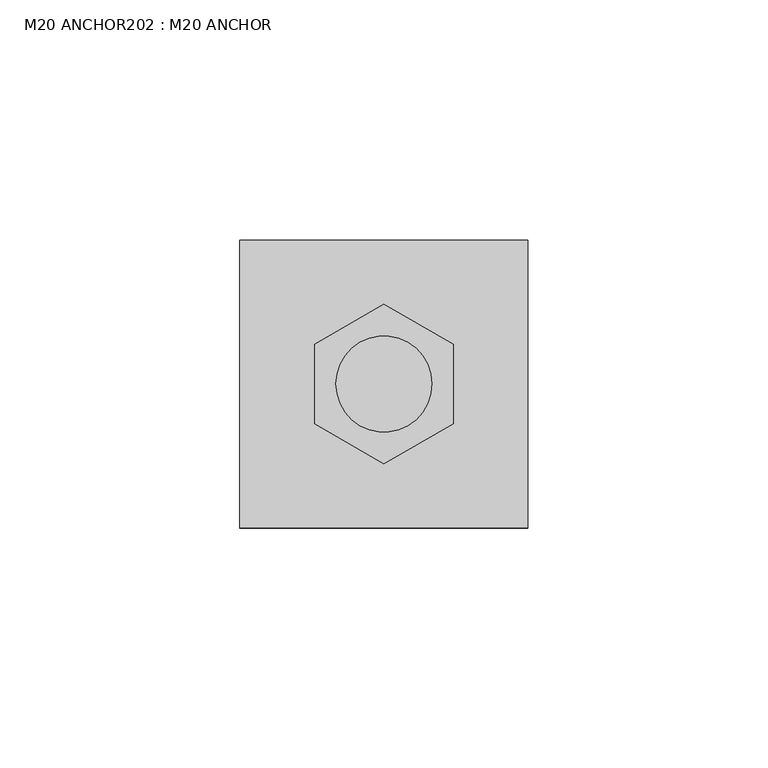
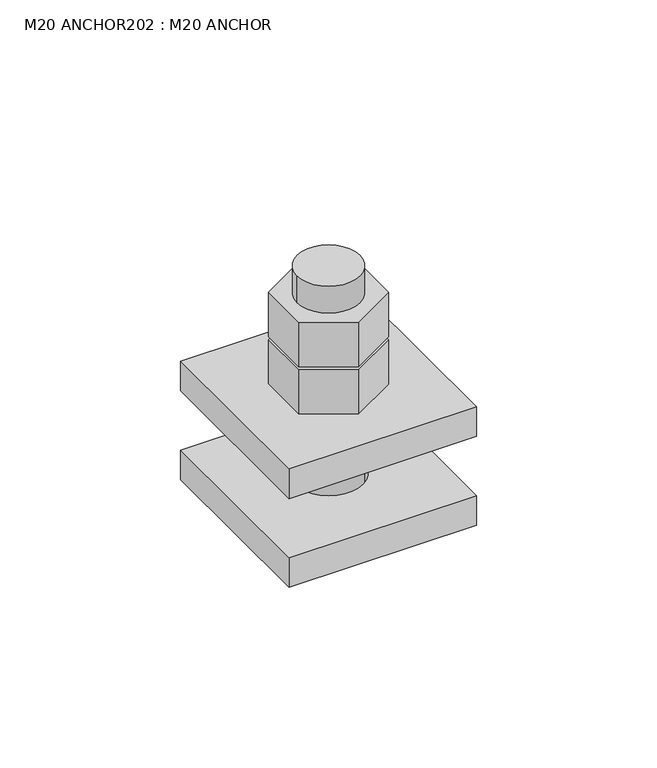
"""IFC4 building model written with IfcOpenShell, lengths in millimetres: fastener geometry, M20 ANCHOR202 : M20 ANCHOR."""

from ifc_helpers import new_model, si_unit, point, frame, frame_2d, origin, place, context, project, spatial, polyline, circle_curve, trimmed, segment, composite_curve, outline, extrude, source, transform, mapped, element, save


def m20_anchor202_m20_anchor_9b2e2336(model_context):
    return source(origin(), model_context, "Body", "SweptSolid", [
        extrude(outline(polyline([(8991.9144032, 22453.9464399), (8977.5062842, 22445.6279085), (8963.0981652, 22453.9464399), (8963.0981652, 22470.5835027), (8977.5062842, 22478.9020341), (8991.9144032, 22470.5835027), (8991.9144032, 22453.9464399)]), holes=[composite_curve([segment(trimmed(circle_curve(frame_2d((8977.5062842, 22462.2649713)), 10.0), [point((8967.5062842, 22462.2649713))], [point((8987.5062842, 22462.2649713))], True, "CARTESIAN"), True, "CONTINUOUS"), segment(trimmed(circle_curve(frame_2d((8977.5062842, 22462.2649713)), 10.0), [point((8987.5062842, 22462.2649713))], [point((8967.5062842, 22462.2649713))], True, "CARTESIAN"), True, "CONTINUOUS")], self_intersect=False)]), frame((0.0, 0.0, 246.0), z_axis=(0.0, 0.0, 1.0), x_axis=(1.0, 0.0, 0.0)), (0.0, 0.0, 1.0), 15.0),
        extrude(outline(polyline([(8991.9144032, 22453.9464399), (8977.5062842, 22445.6279085), (8963.0981652, 22453.9464399), (8963.0981652, 22470.5835027), (8977.5062842, 22478.9020341), (8991.9144032, 22470.5835027), (8991.9144032, 22453.9464399)]), holes=[composite_curve([segment(trimmed(circle_curve(frame_2d((8977.5062842, 22462.2649713)), 10.0), [point((8967.5062842, 22462.2649713))], [point((8987.5062842, 22462.2649713))], True, "CARTESIAN"), True, "CONTINUOUS"), segment(trimmed(circle_curve(frame_2d((8977.5062842, 22462.2649713)), 10.0), [point((8987.5062842, 22462.2649713))], [point((8967.5062842, 22462.2649713))], True, "CARTESIAN"), True, "CONTINUOUS")], self_intersect=False)]), frame((0.0, 0.0, 230.0), z_axis=(0.0, 0.0, 1.0), x_axis=(1.0, 0.0, 0.0)), (0.0, 0.0, 1.0), 15.0),
        extrude(outline(composite_curve([segment(trimmed(circle_curve(frame_2d((8977.5062842, 22462.2649713)), 10.0), [point((8967.5062842, 22462.2649713))], [point((8987.5062842, 22462.2649713))], False, "CARTESIAN"), True, "CONTINUOUS"), segment(trimmed(circle_curve(frame_2d((8977.5062842, 22462.2649713)), 10.0), [point((8987.5062842, 22462.2649713))], [point((8967.5062842, 22462.2649713))], False, "CARTESIAN"), True, "CONTINUOUS")], self_intersect=False)), frame((0.0, 0.0, 190.0), z_axis=(0.0, 0.0, 1.0), x_axis=(1.0, 0.0, 0.0)), (0.0, 0.0, 1.0), 80.0),
        extrude(outline(polyline([(9007.5062842, 22432.2649713), (8947.5062842, 22432.2649713), (8947.5062842, 22492.2649713), (9007.5062842, 22492.2649713), (9007.5062842, 22432.2649713)]), holes=[composite_curve([segment(trimmed(circle_curve(frame_2d((8977.5062842, 22462.2649713)), 11.0), [point((8966.5062842, 22462.2649713))], [point((8988.5062842, 22462.2649713))], True, "CARTESIAN"), True, "CONTINUOUS"), segment(trimmed(circle_curve(frame_2d((8977.5062842, 22462.2649713)), 11.0), [point((8988.5062842, 22462.2649713))], [point((8966.5062842, 22462.2649713))], True, "CARTESIAN"), True, "CONTINUOUS")], self_intersect=False)]), frame((0.0, 0.0, 190.0), z_axis=(0.0, 0.0, 1.0), x_axis=(1.0, 0.0, 0.0)), (0.0, 0.0, 1.0), 10.0),
        extrude(outline(polyline([(9007.5062842, 22432.2649713), (8947.5062842, 22432.2649713), (8947.5062842, 22492.2649713), (9007.5062842, 22492.2649713), (9007.5062842, 22432.2649713)]), holes=[composite_curve([segment(trimmed(circle_curve(frame_2d((8977.5062842, 22462.2649713)), 11.0), [point((8966.5062842, 22462.2649713))], [point((8988.5062842, 22462.2649713))], True, "CARTESIAN"), True, "CONTINUOUS"), segment(trimmed(circle_curve(frame_2d((8977.5062842, 22462.2649713)), 11.0), [point((8988.5062842, 22462.2649713))], [point((8966.5062842, 22462.2649713))], True, "CARTESIAN"), True, "CONTINUOUS")], self_intersect=False)]), frame((0.0, 0.0, 220.0), z_axis=(0.0, 0.0, 1.0), x_axis=(1.0, 0.0, 0.0)), (0.0, 0.0, 1.0), 10.0),
    ])


if __name__ == "__main__":
    model = new_model("IFC4")
    model_context = context("Model", 3, world=origin())
    ifc_project = project(units=[si_unit("LENGTHUNIT", "METRE", prefix="MILLI")], contexts=[model_context])
    site = spatial("IfcSite", under=ifc_project)
    building = spatial("IfcBuilding", under=site)
    placement = place(None, origin())
    m20_anchor202_m20_anchor_shape = m20_anchor202_m20_anchor_9b2e2336(model_context)
    element("IfcFastener", 1, ObjectType="M20 ANCHOR202 : M20 ANCHOR", at=placement, inside=building, context=model_context, shape_type="MappedRepresentation", body=[
        mapped(m20_anchor202_m20_anchor_shape, transform((0.0, 0.0, 0.0), x_axis=(1.0, 0.0, 0.0), y_axis=(0.0, 1.0, 0.0), z_axis=(0.0, 0.0, 1.0))),
    ])
    save(model, "model.ifc")
